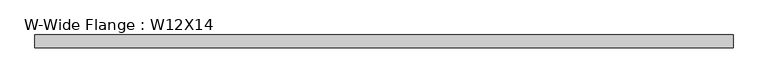
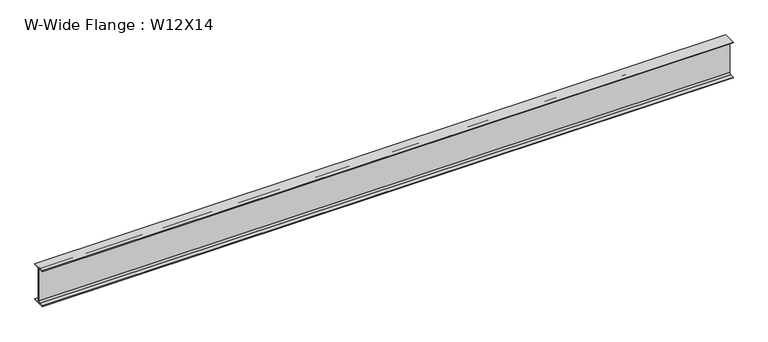
"""IFC4 building model written with IfcOpenShell, lengths in millimetres: beam geometry, W-Wide Flange : W12X14."""

from ifc_helpers import new_model, si_unit, point, frame, frame_2d, origin, place, context, project, spatial, polyline, circle_curve, trimmed, segment, composite_curve, outline, extrude, source, transform, mapped, element, save


def w_wide_flange_w12x14_5d08e082(model_context):
    return source(origin(), model_context, "Body", "SweptSolid", [
        extrude(outline(composite_curve([segment(polyline([(50.419, -145.415), (50.419, -151.13), (-50.419, -151.13), (-50.419, -145.415), (-15.875, -145.415)]), True, "CONTINUOUS"), segment(trimmed(circle_curve(frame_2d((-15.875, -132.08)), 13.335), [point((-15.875, -145.415))], [point((-2.54, -132.08))], True, "CARTESIAN"), True, "CONTINUOUS"), segment(polyline([(-2.54, -132.08), (-2.54, 132.08)]), True, "CONTINUOUS"), segment(trimmed(circle_curve(frame_2d((-15.875, 132.08)), 13.335), [point((-2.54, 132.08))], [point((-15.875, 145.415))], True, "CARTESIAN"), True, "CONTINUOUS"), segment(polyline([(-15.875, 145.415), (-50.419, 145.415), (-50.419, 151.13), (50.419, 151.13), (50.419, 145.415), (15.875, 145.415)]), True, "CONTINUOUS"), segment(trimmed(circle_curve(frame_2d((15.875, 132.08)), 13.335), [point((15.875, 145.415))], [point((2.54, 132.08))], True, "CARTESIAN"), True, "CONTINUOUS"), segment(polyline([(2.54, 132.08), (2.54, -132.08)]), True, "CONTINUOUS"), segment(trimmed(circle_curve(frame_2d((15.875, -132.08)), 13.335), [point((2.54, -132.08))], [point((15.875, -145.415))], True, "CARTESIAN"), True, "CONTINUOUS"), segment(polyline([(15.875, -145.415), (50.419, -145.415)]), True, "CONTINUOUS")], self_intersect=False)), frame((-2769.108, 0.0, 0.0), z_axis=(1.0, 0.0, 0.0), x_axis=(0.0, 1.0, 0.0)), (0.0, 0.0, 1.0), 5538.216),
    ])


if __name__ == "__main__":
    model = new_model("IFC4")
    model_context = context("Model", 3, world=origin())
    ifc_project = project(units=[si_unit("LENGTHUNIT", "METRE", prefix="MILLI")], contexts=[model_context])
    site = spatial("IfcSite", under=ifc_project)
    building = spatial("IfcBuilding", under=site)
    placement = place(None, origin())
    w_wide_flange_w12x14_shape = w_wide_flange_w12x14_5d08e082(model_context)
    element("IfcBeam", 1, ObjectType="W-Wide Flange : W12X14", at=placement, inside=building, context=model_context, shape_type="MappedRepresentation", body=[
        mapped(w_wide_flange_w12x14_shape, transform((0.0, 0.0, 0.0), x_axis=(1.0, 0.0, 0.0), y_axis=(0.0, 1.0, 0.0), z_axis=(0.0, 0.0, 1.0))),
    ])
    save(model, "model.ifc")

# Revit data of these elements
# Type "W-Wide Flange : W12X14"
#   Assembly Code = "B10"
#   W = 14
#   Length [instance default] = 5' - 0"
#   bf = 0' - 3.97"
#   d = 0' - 11.9"
#   k = 0' - 0 3/4"
#   k2 = 0' - 0.525"
#   tf = 0' - 0.225"
#   tw = 0' - 0.2"
#   A = 0.0288889 SF
#   Structural Material [instance default] = Steel ASTM A992
# Element 1 (IfcBeam, "W-Wide Flange : W12X14")
#   Materials on its faces: "Steel ASTM A992"
# Materials
#   "Steel ASTM A992": class "Metal", colour RGB 199 199 199, transparency 0, Description = "Structural steel 50ksi", Cost = 0
